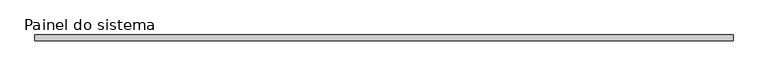
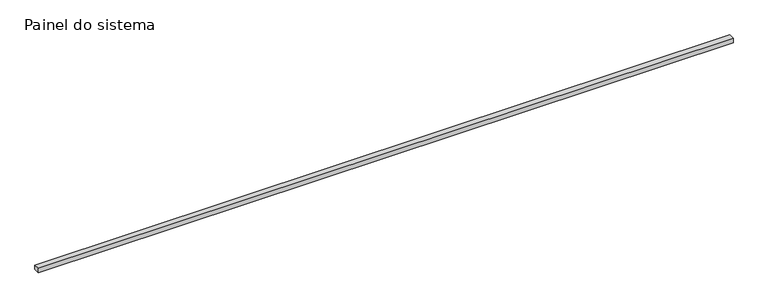
"""IFC4 building model written with IfcOpenShell, lengths in millimetres: plate geometry, Painel do sistema : Envidraçado."""

from ifc_helpers import new_model, si_unit, origin, origin_with_axes, place, context, project, spatial, polyline, outline, extrude, source, transform, mapped, element, save


def painel_do_sistema_1cb3a730(model_context):
    return source(origin(), model_context, "Body", "SweptSolid", [
        extrude(outline(polyline([(1500.0, 24.5), (-1500.0, 24.5), (-1500.0, 49.5), (1500.0, 49.5), (1500.0, 24.5)])), origin_with_axes(), (0.0, 0.0, 1.0), 20.0931032),
    ])


if __name__ == "__main__":
    model = new_model("IFC4")
    model_context = context("Model", 3, world=origin())
    ifc_project = project(units=[si_unit("LENGTHUNIT", "METRE", prefix="MILLI")], contexts=[model_context])
    site = spatial("IfcSite", under=ifc_project)
    building = spatial("IfcBuilding", under=site)
    placement = place(None, origin())
    painel_do_sistema_shape = painel_do_sistema_1cb3a730(model_context)
    element("IfcPlate", 1, ObjectType="Painel do sistema : Envidraçado", at=placement, inside=building, context=model_context, shape_type="MappedRepresentation", body=[
        mapped(painel_do_sistema_shape, transform((0.0, 0.0, 0.0), x_axis=(1.0, 0.0, 0.0), y_axis=(0.0, 1.0, 0.0), z_axis=(0.0, 0.0, 1.0))),
    ])
    save(model, "model.ifc")

# Revit data of these elements
# Type "Painel do sistema : Envidraçado"
#   Construction Type Id = "GSP4R"
#   Analytic Construction = "Vidraça única Pilkington 1/8 pol"
#   Visual Light Transmittance = 0.9
#   Solar Heat Gain Coefficient = 0.86
#   Heat Transfer Coefficient (U) = 6.7069 W/(m²·K)
# Element 1 (IfcPlate, "Painel do sistema : Envidraçado")
#   Materials on its faces: "Vidro"
# Materials
#   "Vidro": class "Vidro", colour RGB 0 128 192, transparency 0.9, Description = "Vidro de sílica", Cost = 0
